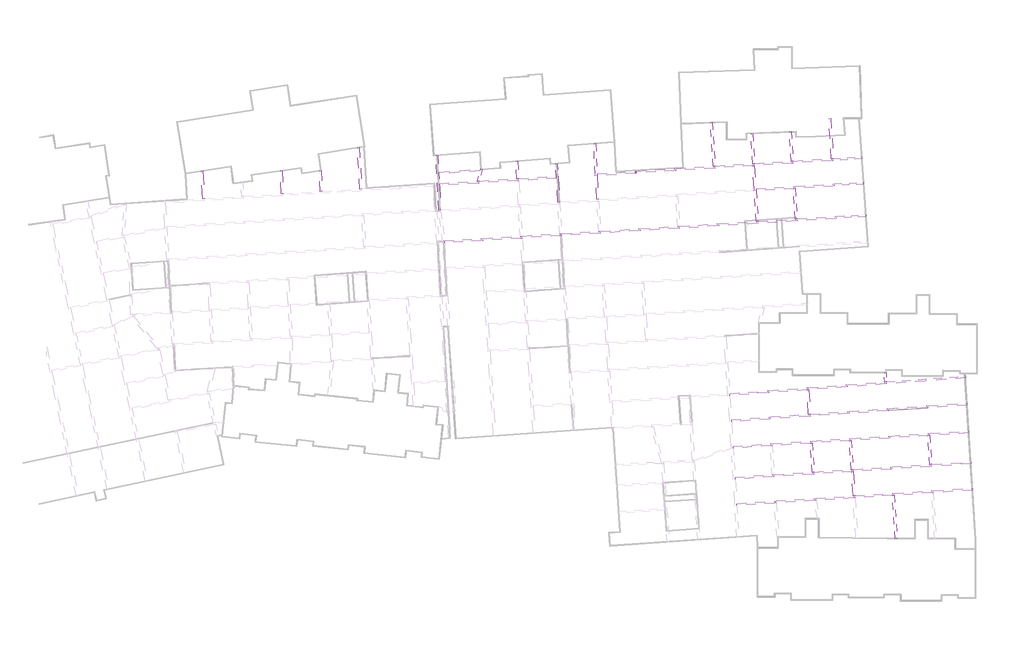
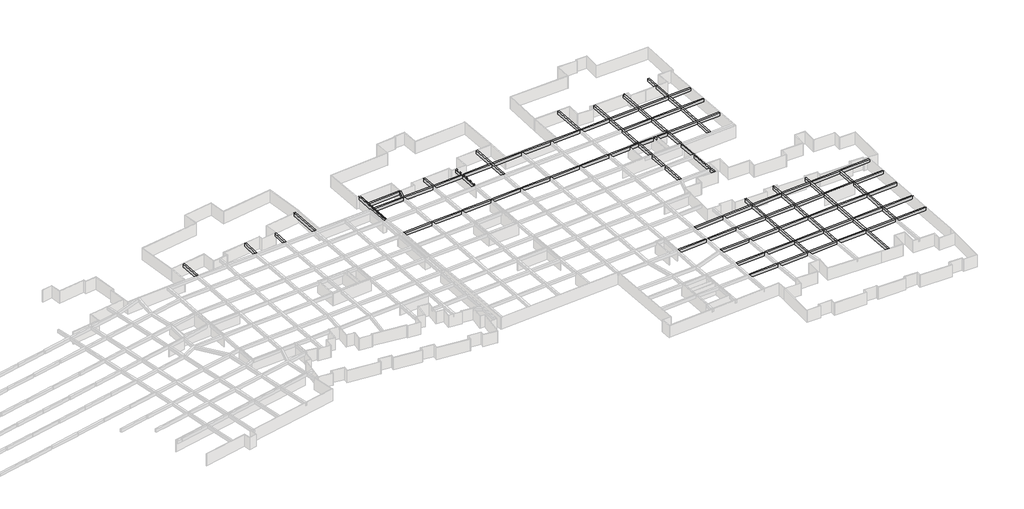
# One storey, part 14 of 14: 33 beams.
"""IFC4 building model written with IfcOpenShell, lengths in millimetres."""

from ifc_helpers import new_model, si_unit, frame, origin, place, context, project, spatial, polyline, outline, extrude, faceted_brep, element, save

model = new_model("IFC4")

# Units and contexts
model_context = context("Model", 3, world=origin())
ifc_project = project(units=[si_unit("LENGTHUNIT", "METRE", prefix="MILLI")], contexts=[model_context])

# Site, building, storey
site = spatial("IfcSite", under=ifc_project)
building = spatial("IfcBuilding", under=site)
storey = spatial("IfcBuildingStorey", under=building, Name="户型图", Elevation=0.0)

# Beams
placement = place(None, origin())
element("IfcBeam", 1, ObjectType="混凝土 - 矩形梁 : KL_beam", at=placement, inside=storey, context=model_context, shape_type="SweptSolid", body=[
    extrude(outline(polyline([(-187005.0921828, -124380.2167121), (-186605.8707912, -124355.2711605), (-186253.1826967, -129999.5894137), (-186652.4040882, -130024.5349652), (-187005.0921828, -124380.2167121)])), frame((0.0, 0.0, 2500.0), z_axis=(0.0, 0.0, 1.0), x_axis=(1.0, 0.0, 0.0)), (0.0, 0.0, 1.0), 800.0),
])
element("IfcBeam", 2, ObjectType="混凝土 - 矩形梁 : KL_beam", at=placement, inside=storey, context=model_context, shape_type="SweptSolid", body=[
    extrude(outline(polyline([(-170857.4371992, -124339.2940821), (-170457.6808684, -124325.3342834), (-170294.3543471, -129002.3939138), (-170693.7267176, -129027.3488993), (-170857.4371992, -124339.2940821)])), frame((0.0, 0.0, 2500.0), z_axis=(0.0, 0.0, 1.0), x_axis=(1.0, 0.0, 0.0)), (0.0, 0.0, 1.0), 800.0),
])
element("IfcBeam", 3, ObjectType="混凝土 - 矩形梁 : KL_beam", at=placement, inside=storey, context=model_context, shape_type="SweptSolid", body=[
    extrude(outline(polyline([(-162964.5535143, -124279.8902248), (-162565.3321228, -124254.9446733), (-162299.8992046, -128502.8563213), (-162699.1205962, -128527.8018729), (-162964.5535143, -124279.8902248)])), frame((0.0, 0.0, 2500.0), z_axis=(0.0, 0.0, 1.0), x_axis=(1.0, 0.0, 0.0)), (0.0, 0.0, 1.0), 800.0),
])
element("IfcBeam", 4, ObjectType="混凝土 - 矩形梁 : KL_beam", at=placement, inside=storey, context=model_context, shape_type="SweptSolid", body=[
    extrude(outline(polyline([(-155213.0308783, -119595.1268602), (-154813.8094867, -119570.1813086), (-154286.932885, -128002.1620485), (-154686.1542765, -128027.1076001), (-155213.0308783, -119595.1268602)])), frame((0.0, 0.0, 2500.0), z_axis=(0.0, 0.0, 1.0), x_axis=(1.0, 0.0, 0.0)), (0.0, 0.0, 1.0), 800.0),
])
element("IfcBeam", 5, ObjectType="混凝土 - 矩形梁 : KL_beam", at=placement, inside=storey, context=model_context, shape_type="Brep", body=[
    faceted_brep([(-52374.3043839, -126618.4184989, 3300.0), (-52349.2555626, -127017.6334242, 3300.0), (-52349.2555626, -127017.6334242, 2500.0), (-52374.3043839, -126618.4184989, 2500.0), (-58173.9130136, -126982.3161169, 3300.0), (-58573.1279522, -127007.3649391, 3300.0), (-66248.800325, -127488.9765565, 3300.0), (-66648.0254552, -127514.0260182, 3300.0), (-74177.9187714, -127986.4906992, 3300.0), (-74150.0154686, -128385.5265194, 3300.0), (-66620.1221525, -127913.0618384, 3300.0), (-66220.8970222, -127888.0123768, 3300.0), (-58548.1823998, -127406.586344, 3300.0), (-58148.9674612, -127381.5375218, 3300.0), (-74150.0154686, -128385.5265194, 2500.0), (-66620.1221525, -127913.0618384, 2500.0), (-66220.8970222, -127888.0123768, 2500.0), (-58548.1823998, -127406.586344, 2500.0), (-58148.9674612, -127381.5375218, 2500.0), (-74177.9187714, -127986.4906992, 2500.0), (-66648.0254552, -127514.0260182, 2500.0), (-66248.800325, -127488.9765565, 2500.0), (-58573.1279522, -127007.3649391, 2500.0), (-58173.9130136, -126982.3161169, 2500.0)], [[[0, 1, 2, 3]], [[1, 0, 4, 5, 6, 7, 8, 9, 10, 11, 12, 13]], [[2, 1, 13, 12, 11, 10, 9, 14, 15, 16, 17, 18]], [[3, 2, 18, 17, 16, 15, 14, 19, 20, 21, 22, 23]], [[0, 3, 23, 22, 21, 20, 19, 8, 7, 6, 5, 4]], [[8, 19, 14, 9]]]),
])
element("IfcBeam", 6, ObjectType="混凝土 - 矩形梁 : KL_beam", at=placement, inside=storey, context=model_context, shape_type="Brep", body=[
    faceted_brep([(-51938.8314526, -133222.3446571, 3300.0), (-51913.8859011, -133621.5660486, 3300.0), (-51913.8859011, -133621.5660486, 2500.0), (-51938.8314526, -133222.3446571, 2500.0), (-57761.268311, -133586.1625832, 3300.0), (-58160.4897025, -133611.1081347, 3300.0), (-65787.374178, -134087.6778873, 3300.0), (-66186.6065264, -134112.6241234, 3300.0), (-73716.6359875, -134583.1418412, 3300.0), (-74115.868336, -134608.0880774, 3300.0), (-81725.5469195, -135083.582711, 3300.0), (-82124.7687178, -135108.5282879, 3300.0), (-89692.9705485, -135581.4312256, 3300.0), (-90092.1926208, -135606.3768197, 3300.0), (-97677.4119955, -136080.3431072, 3300.0), (-98076.6340678, -136105.2887013, 3300.0), (-105753.707815, -136584.9945559, 3300.0), (-106152.9326387, -136609.9403219, 3300.0), (-113651.9046068, -137078.5173964, 3300.0), (-114051.1259984, -137103.462948, 3300.0), (-121674.9817155, -137579.843447, 3300.0), (-122074.2065392, -137604.789213, 3300.0), (-129690.7407312, -138080.7122228, 3300.0), (-130089.9623439, -138105.6577881, 3300.0), (-137513.7217746, -138569.535169, 3300.0), (-137466.852736, -138967.3866603, 3300.0), (-130064.5965359, -138504.8529197, 3300.0), (-129665.3749232, -138479.9073544, 3300.0), (-122048.4315655, -138003.9587776, 3300.0), (-121649.210174, -137979.0132261, 3300.0), (-114026.1804468, -137502.6843395, 3300.0), (-113626.9590553, -137477.738788, 3300.0), (-106126.3316752, -137009.0582742, 3300.0), (-105727.1068515, -136984.1125082, 3300.0), (-98050.9512296, -136504.4640231, 3300.0), (-97651.7291573, -136479.518429, 3300.0), (-90066.5097827, -136005.5521415, 3300.0), (-89667.2877103, -135980.6065474, 3300.0), (-82099.2532336, -135507.7140669, 3300.0), (-81700.0314352, -135482.76849, 3300.0), (-74087.9649807, -135007.124649, 3300.0), (-73688.7326322, -134982.1784128, 3300.0), (-66158.7031711, -134511.6606951, 3300.0), (-65759.4708227, -134486.7144589, 3300.0), (-58135.544151, -134010.3295263, 3300.0), (-57736.3227594, -133985.3839747, 3300.0), (-137466.852736, -138967.3866603, 2500.0), (-130064.5965359, -138504.8529197, 2500.0), (-129665.3749232, -138479.9073544, 2500.0), (-122048.4315655, -138003.9587776, 2500.0), (-121649.210174, -137979.0132261, 2500.0), (-114026.1804468, -137502.6843395, 2500.0), (-113626.9590553, -137477.738788, 2500.0), (-106126.3316752, -137009.0582742, 2500.0), (-105727.1068515, -136984.1125082, 2500.0), (-98050.9512296, -136504.4640231, 2500.0), (-97651.7291573, -136479.518429, 2500.0), (-90066.5097827, -136005.5521415, 2500.0), (-89667.2877103, -135980.6065474, 2500.0), (-82099.2532336, -135507.7140669, 2500.0), (-81700.0314352, -135482.76849, 2500.0), (-74087.9649807, -135007.124649, 2500.0), (-73688.7326322, -134982.1784128, 2500.0), (-66158.7031711, -134511.6606951, 2500.0), (-65759.4708227, -134486.7144589, 2500.0), (-58135.544151, -134010.3295263, 2500.0), (-57736.3227594, -133985.3839747, 2500.0), (-137513.7217746, -138569.535169, 2500.0), (-130089.9623439, -138105.6577881, 2500.0), (-129690.7407312, -138080.7122228, 2500.0), (-122074.2065392, -137604.789213, 2500.0), (-121674.9817155, -137579.843447, 2500.0), (-114051.1259984, -137103.462948, 2500.0), (-113651.9046068, -137078.5173964, 2500.0), (-106152.9326387, -136609.9403219, 2500.0), (-105753.707815, -136584.9945559, 2500.0), (-98076.6340678, -136105.2887013, 2500.0), (-97677.4119955, -136080.3431072, 2500.0), (-90092.1926208, -135606.3768197, 2500.0), (-89692.9705485, -135581.4312256, 2500.0), (-82124.7687178, -135108.5282879, 2500.0), (-81725.5469195, -135083.582711, 2500.0), (-74115.868336, -134608.0880774, 2500.0), (-73716.6359875, -134583.1418412, 2500.0), (-66186.6065264, -134112.6241234, 2500.0), (-65787.374178, -134087.6778873, 2500.0), (-58160.4897025, -133611.1081347, 2500.0), (-57761.268311, -133586.1625832, 2500.0)], [[[0, 1, 2, 3]], [[1, 0, 4, 5, 6, 7, 8, 9, 10, 11, 12, 13, 14, 15, 16, 17, 18, 19, 20, 21, 22, 23, 24, 25, 26, 27, 28, 29, 30, 31, 32, 33, 34, 35, 36, 37, 38, 39, 40, 41, 42, 43, 44, 45]], [[2, 1, 45, 44, 43, 42, 41, 40, 39, 38, 37, 36, 35, 34, 33, 32, 31, 30, 29, 28, 27, 26, 25, 46, 47, 48, 49, 50, 51, 52, 53, 54, 55, 56, 57, 58, 59, 60, 61, 62, 63, 64, 65, 66]], [[3, 2, 66, 65, 64, 63, 62, 61, 60, 59, 58, 57, 56, 55, 54, 53, 52, 51, 50, 49, 48, 47, 46, 67, 68, 69, 70, 71, 72, 73, 74, 75, 76, 77, 78, 79, 80, 81, 82, 83, 84, 85, 86, 87]], [[0, 3, 87, 86, 85, 84, 83, 82, 81, 80, 79, 78, 77, 76, 75, 74, 73, 72, 71, 70, 69, 68, 67, 24, 23, 22, 21, 20, 19, 18, 17, 16, 15, 14, 13, 12, 11, 10, 9, 8, 7, 6, 5, 4]], [[25, 24, 67, 46]]]),
])
element("IfcBeam", 7, ObjectType="混凝土 - 矩形梁 : KL_beam", at=placement, inside=storey, context=model_context, shape_type="Brep", body=[
    faceted_brep([(-129842.1738274, -124027.4632209, 3300.0), (-130231.923834, -123937.491379, 3300.0), (-130326.1623243, -124345.7241266, 3300.0), (-130806.4572254, -126426.3188663, 3300.0), (-130389.9881583, -126400.5461175, 3300.0), (-129842.1738274, -124027.4632209, 2500.0), (-130389.9881583, -126400.5461175, 2500.0), (-130231.923834, -123937.491379, 2500.0), (-130806.4572254, -126426.3188663, 2500.0), (-130326.1623243, -124345.7241266, 2500.0)], [[[0, 1, 2, 3, 4]], [[5, 0, 4, 6]], [[7, 5, 6, 8, 9]], [[1, 7, 9, 8, 3, 2]], [[4, 3, 8, 6]], [[1, 0, 5, 7]]]),
])
element("IfcBeam", 8, ObjectType="混凝土 - 矩形梁 : KL_beam", at=placement, inside=storey, context=model_context, shape_type="SweptSolid", body=[
    extrude(outline(polyline([(-123047.7665845, -122325.8850296), (-122648.896806, -122295.8367384), (-122377.03025, -125904.6726724), (-122776.3022919, -125929.3812014), (-123047.7665845, -122325.8850296)])), frame((0.0, 0.0, 2500.0), z_axis=(0.0, 0.0, 1.0), x_axis=(1.0, 0.0, 0.0)), (0.0, 0.0, 1.0), 800.0),
])
element("IfcBeam", 9, ObjectType="混凝土 - 矩形梁 : KL_beam", at=placement, inside=storey, context=model_context, shape_type="Brep", body=[
    faceted_brep([(-114574.1543033, -122851.64996, 3300.0), (-114574.1543033, -122851.64996, 2500.0), (-114973.2688243, -122878.2506949, 2500.0), (-114973.2688243, -122878.2506949, 3300.0), (-114802.7997937, -125435.9494127, 3300.0), (-114776.1987592, -125835.0684284, 3300.0), (-114453.9509255, -130670.0397306, 3300.0), (-114054.8364044, -130643.4389957, 3300.0), (-114376.9579948, -125810.3618349, 3300.0), (-114403.5590293, -125411.2428193, 3300.0), (-114802.7997937, -125435.9494127, 2500.0), (-114776.1987592, -125835.0684284, 2500.0), (-114453.9509255, -130670.0397306, 2500.0), (-114403.5590293, -125411.2428193, 2500.0), (-114376.9579948, -125810.3618349, 2500.0), (-114054.8364044, -130643.4389957, 2500.0)], [[[0, 1, 2, 3]], [[0, 3, 4, 5, 6, 7, 8, 9]], [[3, 2, 10, 11, 12, 6, 5, 4]], [[2, 1, 13, 14, 15, 12, 11, 10]], [[1, 0, 9, 8, 7, 15, 14, 13]], [[7, 6, 12, 15]]]),
])
element("IfcBeam", 10, ObjectType="混凝土 - 矩形梁 : KL_beam", at=placement, inside=storey, context=model_context, shape_type="Brep", body=[
    faceted_brep([(-107176.9227789, -118773.8861583, 3300.0), (-106777.470965, -118752.9517758, 3300.0), (-106777.470965, -118752.9517758, 2500.0), (-107176.9227789, -118773.8861583, 2500.0), (-106853.5598144, -124944.0190844, 3300.0), (-106832.624498, -125343.488717, 3300.0), (-106580.971679, -130145.3105546, 3300.0), (-106181.8169664, -130118.707141, 3300.0), (-106433.3957536, -125318.2979156, 3300.0), (-106454.3316163, -124918.8178582, 3300.0), (-106181.8169664, -130118.707141, 2500.0), (-106433.3957536, -125318.2979156, 2500.0), (-106454.3316163, -124918.8178582, 2500.0), (-106580.971679, -130145.3105546, 2500.0), (-106832.624498, -125343.488717, 2500.0), (-106853.5598144, -124944.0190844, 2500.0)], [[[0, 1, 2, 3]], [[1, 0, 4, 5, 6, 7, 8, 9]], [[2, 1, 9, 8, 7, 10, 11, 12]], [[3, 2, 12, 11, 10, 13, 14, 15]], [[0, 3, 15, 14, 13, 6, 5, 4]], [[7, 6, 13, 10]]]),
])
element("IfcBeam", 11, ObjectType="混凝土 - 矩形梁 : KL_beam", at=placement, inside=storey, context=model_context, shape_type="Brep", body=[
    faceted_brep([(-31634.7856178, -166005.21398, 3300.0), (-31604.8822978, -166404.0946532, 3300.0), (-31604.8822978, -166404.0946532, 2500.0), (-31634.7856178, -166005.21398, 2500.0), (-47623.313796, -167203.8433097, 3300.0), (-48022.1944692, -167233.7466297, 3300.0), (-55561.2153478, -167798.9325831, 3300.0), (-55960.1119301, -167828.8370958, 3300.0), (-63527.0942157, -168396.1192624, 3300.0), (-63925.978016, -168426.0228168, 3300.0), (-71553.260966, -168997.8256086, 3300.0), (-71952.1673161, -169027.7308535, 3300.0), (-79519.6147606, -169595.0478922, 3300.0), (-79494.0977596, -169994.2573993, 3300.0), (-71926.7900008, -169426.9508326, 3300.0), (-71527.8836507, -169397.0455877, 3300.0), (-63897.65415, -168825.0218986, 3300.0), (-63498.7703497, -168795.1183442, 3300.0), (-55933.7711758, -168227.9848477, 3300.0), (-55534.8745936, -168198.0803351, 3300.0), (-47994.1941782, -167632.7699693, 3300.0), (-47595.2955182, -167602.8653009, 3300.0), (-39950.5556653, -167029.7537985, 3300.0), (-39551.6447709, -166999.8482129, 3300.0), (-79494.0977596, -169994.2573993, 2500.0), (-71926.7900008, -169426.9508326, 2500.0), (-71527.8836507, -169397.0455877, 2500.0), (-63897.65415, -168825.0218986, 2500.0), (-63498.7703497, -168795.1183442, 2500.0), (-55933.7711758, -168227.9848477, 2500.0), (-55534.8745936, -168198.0803351, 2500.0), (-47994.1941782, -167632.7699693, 2500.0), (-47595.2955182, -167602.8653009, 2500.0), (-39950.5556653, -167029.7537985, 2500.0), (-39551.6447709, -166999.8482129, 2500.0), (-79519.6147606, -169595.0478922, 2500.0), (-71952.1673161, -169027.7308535, 2500.0), (-71553.260966, -168997.8256086, 2500.0), (-63925.978016, -168426.0228168, 2500.0), (-63527.0942157, -168396.1192624, 2500.0), (-55960.1119301, -167828.8370958, 2500.0), (-55561.2153478, -167798.9325831, 2500.0), (-48022.1944692, -167233.7466297, 2500.0), (-47623.313796, -167203.8433097, 2500.0)], [[[0, 1, 2, 3]], [[1, 0, 4, 5, 6, 7, 8, 9, 10, 11, 12, 13, 14, 15, 16, 17, 18, 19, 20, 21, 22, 23]], [[2, 1, 23, 22, 21, 20, 19, 18, 17, 16, 15, 14, 13, 24, 25, 26, 27, 28, 29, 30, 31, 32, 33, 34]], [[3, 2, 34, 33, 32, 31, 30, 29, 28, 27, 26, 25, 24, 35, 36, 37, 38, 39, 40, 41, 42, 43]], [[0, 3, 43, 42, 41, 40, 39, 38, 37, 36, 35, 12, 11, 10, 9, 8, 7, 6, 5, 4]], [[12, 35, 24, 13]]]),
])
element("IfcBeam", 12, ObjectType="混凝土 - 矩形梁 : KL_beam", at=placement, inside=storey, context=model_context, shape_type="Brep", body=[
    faceted_brep([(-106832.624498, -125343.488717, 3300.0), (-106853.5598144, -124944.0190844, 3300.0), (-114403.5590293, -125411.2428193, 3300.0), (-114376.9579948, -125810.3618349, 3300.0), (-106832.624498, -125343.488717, 2500.0), (-114376.9579948, -125810.3618349, 2500.0), (-106853.5598144, -124944.0190844, 2500.0), (-114403.5590293, -125411.2428193, 2500.0)], [[[0, 1, 2, 3]], [[4, 0, 3, 5]], [[6, 4, 5, 7]], [[1, 6, 7, 2]], [[1, 0, 4, 6]], [[3, 2, 7, 5]]]),
    faceted_brep([(-114802.7997937, -125435.9494127, 3300.0), (-114776.1987592, -125835.0684284, 3300.0), (-114776.1987592, -125835.0684284, 2500.0), (-114802.7997937, -125435.9494127, 2500.0), (-122377.03025, -125904.6726724, 3300.0), (-122776.3022919, -125929.3812014, 3300.0), (-130389.9881583, -126400.5461175, 3300.0), (-130806.4572254, -126426.3188663, 3300.0), (-138525.1741329, -126903.9835175, 3300.0), (-138504.2388166, -127303.4531502, 3300.0), (-130806.6290639, -126827.0946929, 3300.0), (-130407.3922508, -126802.388344, 3300.0), (-122753.4617992, -126328.7329342, 3300.0), (-122354.2077216, -126304.0255169, 3300.0), (-138504.2388166, -127303.4531502, 2500.0), (-130806.6290639, -126827.0946929, 2500.0), (-130407.3922508, -126802.388344, 2500.0), (-122753.4617992, -126328.7329342, 2500.0), (-122354.2077216, -126304.0255169, 2500.0), (-138525.1741329, -126903.9835175, 2500.0), (-130806.4572254, -126426.3188663, 2500.0), (-130389.9881583, -126400.5461175, 2500.0), (-122776.3022919, -125929.3812014, 2500.0), (-122377.03025, -125904.6726724, 2500.0)], [[[0, 1, 2, 3]], [[1, 0, 4, 5, 6, 7, 8, 9, 10, 11, 12, 13]], [[2, 1, 13, 12, 11, 10, 9, 14, 15, 16, 17, 18]], [[3, 2, 18, 17, 16, 15, 14, 19, 20, 21, 22, 23]], [[0, 3, 23, 22, 21, 20, 19, 8, 7, 6, 5, 4]], [[9, 8, 19, 14]]]),
])
element("IfcBeam", 13, ObjectType="混凝土 - 矩形梁 : KL_beam", at=placement, inside=storey, context=model_context, shape_type="Brep", body=[
    faceted_brep([(-98647.1108371, -124817.3303339, 3300.0), (-98649.2821204, -124783.5831797, 3300.0), (-98672.7936315, -124418.1556929, 3300.0), (-98827.9389787, -124428.1377049, 3300.0), (-106454.3316163, -124918.8178582, 3300.0), (-106433.3957536, -125318.2979156, 3300.0), (-98802.2561843, -124827.3123459, 3300.0), (-98647.1108371, -124817.3303339, 2500.0), (-106433.3957536, -125318.2979156, 2500.0), (-98802.2561843, -124827.3123459, 2500.0), (-98672.7936315, -124418.1556929, 2500.0), (-98649.2821204, -124783.5831797, 2500.0), (-106454.3316163, -124918.8178582, 2500.0), (-98827.9389787, -124428.1377049, 2500.0)], [[[0, 1, 2, 3, 4, 5, 6]], [[7, 0, 6, 5, 8, 9]], [[10, 11, 7, 9, 8, 12, 13]], [[2, 10, 13, 12, 4, 3]], [[5, 4, 12, 8]], [[2, 1, 0, 7, 11, 10]]]),
])
element("IfcBeam", 14, ObjectType="混凝土 - 矩形梁 : KL_beam", at=placement, inside=storey, context=model_context, shape_type="SweptSolid", body=[
    extrude(outline(polyline([(-130231.923834, -123937.491379), (-130326.1623243, -124345.7241266), (-138626.4766377, -124971.0165776), (-138647.4164777, -124571.4606268), (-130231.923834, -123937.491379)])), frame((0.0, 0.0, 2500.0), z_axis=(0.0, 0.0, 1.0), x_axis=(1.0, 0.0, 0.0)), (0.0, 0.0, 1.0), 800.0),
])
element("IfcBeam", 15, ObjectType="混凝土 - 矩形梁 : KL_beam", at=placement, inside=storey, context=model_context, shape_type="Brep", body=[
    faceted_brep([(-52735.750442, -121456.1127854, 3300.0), (-52710.3049507, -121855.3026237, 3300.0), (-52710.3049507, -121855.3026237, 2500.0), (-52735.750442, -121456.1127854, 2500.0), (-58496.276443, -121823.3050331, 3300.0), (-58895.4665943, -121848.7505443, 3300.0), (-66607.5973218, -122340.3436063, 3300.0), (-67006.78716, -122365.7890976, 3300.0), (-74491.5966275, -122842.8920585, 3300.0), (-74890.7864658, -122868.3375498, 3300.0), (-82475.3933928, -123351.8018835, 3300.0), (-82874.5832311, -123377.2473747, 3300.0), (-90447.1281157, -123859.9428397, 3300.0), (-90846.3180245, -123885.3883354, 3300.0), (-98430.9262918, -124368.8527546, 3300.0), (-98674.8462654, -124384.4009048, 3300.0), (-98672.6950439, -124418.1493498, 3300.0), (-98649.4007742, -124783.590743, 3300.0), (-98405.2434928, -124768.0274662, 3300.0), (-90820.6352256, -124284.563047, 3300.0), (-90421.4453168, -124259.1175513, 3300.0), (-82849.1027592, -123776.4349832, 3300.0), (-82449.9129148, -123750.9894916, 3300.0), (-74908.6843946, -123270.2902204, 3300.0), (-74509.4869911, -123244.8442469, 3300.0), (-66980.1166378, -122764.9008489, 3300.0), (-66580.9192344, -122739.4548754, 3300.0), (-58870.5210232, -122247.9722489, 3300.0), (-58471.3308719, -122222.5267377, 3300.0), (-98649.4007742, -124783.590743, 2500.0), (-98405.2434928, -124768.0274662, 2500.0), (-90820.6352256, -124284.563047, 2500.0), (-90421.4453168, -124259.1175513, 2500.0), (-82849.1027592, -123776.4349832, 2500.0), (-82449.9129148, -123750.9894916, 2500.0), (-74908.6843946, -123270.2902204, 2500.0), (-74509.4869911, -123244.8442469, 2500.0), (-66980.1166378, -122764.9008489, 2500.0), (-66580.9192344, -122739.4548754, 2500.0), (-58870.5210232, -122247.9722489, 2500.0), (-58471.3308719, -122222.5267377, 2500.0), (-98672.6950439, -124418.1493498, 2500.0), (-98674.8462654, -124384.4009048, 2500.0), (-98430.9262918, -124368.8527546, 2500.0), (-90846.3180245, -123885.3883354, 2500.0), (-90447.1281157, -123859.9428397, 2500.0), (-82874.5832311, -123377.2473747, 2500.0), (-82475.3933928, -123351.8018835, 2500.0), (-74890.7864658, -122868.3375498, 2500.0), (-74491.5966275, -122842.8920585, 2500.0), (-67006.78716, -122365.7890976, 2500.0), (-66607.5973218, -122340.3436063, 2500.0), (-58895.4665943, -121848.7505443, 2500.0), (-58496.276443, -121823.3050331, 2500.0)], [[[0, 1, 2, 3]], [[1, 0, 4, 5, 6, 7, 8, 9, 10, 11, 12, 13, 14, 15, 16, 17, 18, 19, 20, 21, 22, 23, 24, 25, 26, 27, 28]], [[2, 1, 28, 27, 26, 25, 24, 23, 22, 21, 20, 19, 18, 17, 29, 30, 31, 32, 33, 34, 35, 36, 37, 38, 39, 40]], [[3, 2, 40, 39, 38, 37, 36, 35, 34, 33, 32, 31, 30, 29, 41, 42, 43, 44, 45, 46, 47, 48, 49, 50, 51, 52, 53]], [[0, 3, 53, 52, 51, 50, 49, 48, 47, 46, 45, 44, 43, 42, 15, 14, 13, 12, 11, 10, 9, 8, 7, 6, 5, 4]], [[15, 42, 41, 29, 17, 16]]]),
])
element("IfcBeam", 16, ObjectType="混凝土 - 矩形梁 : KL_beam", at=placement, inside=storey, context=model_context, shape_type="SweptSolid", body=[
    extrude(outline(polyline([(-83442.4636616, -114468.3174988), (-83043.2738233, -114442.8720075), (-82475.3933928, -123351.8018835), (-82874.5832311, -123377.2473747), (-83442.4636616, -114468.3174988)])), frame((0.0, 0.0, 2500.0), z_axis=(0.0, 0.0, 1.0), x_axis=(1.0, 0.0, 0.0)), (0.0, 0.0, 1.0), 800.0),
])
element("IfcBeam", 17, ObjectType="混凝土 - 矩形梁 : KL_beam", at=placement, inside=storey, context=model_context, shape_type="SweptSolid", body=[
    extrude(outline(polyline([(-75277.2537161, -116805.42457), (-74878.0638779, -116779.9790787), (-74491.5966275, -122842.8920585), (-74890.7864658, -122868.3375498), (-75277.2537161, -116805.42457)])), frame((0.0, 0.0, 2500.0), z_axis=(0.0, 0.0, 1.0), x_axis=(1.0, 0.0, 0.0)), (0.0, 0.0, 1.0), 800.0),
])
element("IfcBeam", 18, ObjectType="混凝土 - 矩形梁 : KL_beam", at=placement, inside=storey, context=model_context, shape_type="SweptSolid", body=[
    extrude(outline(polyline([(-67390.2618088, -116349.8241659), (-66991.0719705, -116324.3786746), (-66607.5973218, -122340.3436063), (-67006.78716, -122365.7890976), (-67390.2618088, -116349.8241659)])), frame((0.0, 0.0, 2500.0), z_axis=(0.0, 0.0, 1.0), x_axis=(1.0, 0.0, 0.0)), (0.0, 0.0, 1.0), 800.0),
])
element("IfcBeam", 19, ObjectType="混凝土 - 矩形梁 : KL_beam", at=placement, inside=storey, context=model_context, shape_type="SweptSolid", body=[
    extrude(outline(polyline([(-59405.2866368, -113689.7380459), (-59006.0652453, -113664.7924943), (-58496.276443, -121823.3050331), (-58895.4665943, -121848.7505443), (-59405.2866368, -113689.7380459)])), frame((0.0, 0.0, 2500.0), z_axis=(0.0, 0.0, 1.0), x_axis=(1.0, 0.0, 0.0)), (0.0, 0.0, 1.0), 800.0),
    extrude(outline(polyline([(-57425.127004, -138965.6708341), (-57824.3483955, -138990.6163857), (-58135.544151, -134010.3295263), (-57736.3227594, -133985.3839747), (-57425.127004, -138965.6708341)])), frame((0.0, 0.0, 2500.0), z_axis=(0.0, 0.0, 1.0), x_axis=(1.0, 0.0, 0.0)), (0.0, 0.0, 1.0), 800.0),
    extrude(outline(polyline([(-58548.1823998, -127406.586344), (-58148.9674612, -127381.5375218), (-57761.268311, -133586.1625832), (-58160.4897025, -133611.1081347), (-58548.1823998, -127406.586344)])), frame((0.0, 0.0, 2500.0), z_axis=(0.0, 0.0, 1.0), x_axis=(1.0, 0.0, 0.0)), (0.0, 0.0, 1.0), 800.0),
    extrude(outline(polyline([(-58173.9130136, -126982.3161169), (-58573.1279522, -127007.3649391), (-58870.5210232, -122247.9722489), (-58471.3308719, -122222.5267377), (-58173.9130136, -126982.3161169)])), frame((0.0, 0.0, 2500.0), z_axis=(0.0, 0.0, 1.0), x_axis=(1.0, 0.0, 0.0)), (0.0, 0.0, 1.0), 800.0),
])
element("IfcBeam", 20, ObjectType="混凝土 - 矩形梁 : KL_beam", at=placement, inside=storey, context=model_context, shape_type="SweptSolid", body=[
    extrude(outline(polyline([(-64460.4085886, -153064.1699143), (-64859.4342087, -153092.0725038), (-64959.6104423, -151659.4856204), (-64560.4102838, -151634.0790467), (-64460.4085886, -153064.1699143)])), frame((0.0, 0.0, 2500.0), z_axis=(0.0, 0.0, 1.0), x_axis=(1.0, 0.0, 0.0)), (0.0, 0.0, 1.0), 800.0),
    extrude(outline(polyline([(-66980.1166378, -122764.9008489), (-66580.9192344, -122739.4548754), (-66248.800325, -127488.9765565), (-66648.0254552, -127514.0260182), (-66980.1166378, -122764.9008489)])), frame((0.0, 0.0, 2500.0), z_axis=(0.0, 0.0, 1.0), x_axis=(1.0, 0.0, 0.0)), (0.0, 0.0, 1.0), 800.0),
    extrude(outline(polyline([(-66620.1221525, -127913.0618384), (-66220.8970222, -127888.0123768), (-65787.374178, -134087.6778873), (-66186.6065264, -134112.6241234), (-66620.1221525, -127913.0618384)])), frame((0.0, 0.0, 2500.0), z_axis=(0.0, 0.0, 1.0), x_axis=(1.0, 0.0, 0.0)), (0.0, 0.0, 1.0), 800.0),
    extrude(outline(polyline([(-66158.7031711, -134511.6606951), (-65759.4708227, -134486.7144589), (-65411.3764652, -139464.6956904), (-65810.6088137, -139489.6419266), (-66158.7031711, -134511.6606951)])), frame((0.0, 0.0, 2500.0), z_axis=(0.0, 0.0, 1.0), x_axis=(1.0, 0.0, 0.0)), (0.0, 0.0, 1.0), 800.0),
    extrude(outline(polyline([(-65782.7054584, -139888.6784983), (-65383.4731099, -139863.7322621), (-65042.807434, -144735.4783979), (-65442.0397825, -144760.4246341), (-65782.7054584, -139888.6784983)])), frame((0.0, 0.0, 2500.0), z_axis=(0.0, 0.0, 1.0), x_axis=(1.0, 0.0, 0.0)), (0.0, 0.0, 1.0), 800.0),
    extrude(outline(polyline([(-65414.1364272, -145159.4612058), (-65014.9040787, -145134.5149696), (-64588.3134192, -151235.04562), (-64987.5135777, -151260.4521937), (-65414.1364272, -145159.4612058)])), frame((0.0, 0.0, 2500.0), z_axis=(0.0, 0.0, 1.0), x_axis=(1.0, 0.0, 0.0)), (0.0, 0.0, 1.0), 800.0),
])
element("IfcBeam", 21, ObjectType="混凝土 - 矩形梁 : KL_beam", at=placement, inside=storey, context=model_context, shape_type="Brep", body=[
    faceted_brep([(-74509.4869911, -123244.8442469, 3300.0), (-74908.6843946, -123270.2902204, 3300.0), (-74577.0927331, -128012.2719042, 3300.0), (-74549.1899952, -128411.2996475, 3300.0), (-74115.868336, -134608.0880774, 3300.0), (-73716.6359875, -134583.1418412, 3300.0), (-74150.0154686, -128385.5265194, 3300.0), (-74177.9187714, -127986.4906992, 3300.0), (-74509.4869911, -123244.8442469, 2500.0), (-73716.6359875, -134583.1418412, 2500.0), (-74150.0154686, -128385.5265194, 2500.0), (-74177.9187714, -127986.4906992, 2500.0), (-74908.6843946, -123270.2902204, 2500.0), (-74115.868336, -134608.0880774, 2500.0), (-74549.1899952, -128411.2996475, 2500.0), (-74577.0927331, -128012.2719042, 2500.0)], [[[0, 1, 2, 3, 4, 5, 6, 7]], [[8, 0, 7, 6, 5, 9, 10, 11]], [[12, 8, 11, 10, 9, 13, 14, 15]], [[1, 12, 15, 14, 13, 4, 3, 2]], [[1, 0, 8, 12]], [[5, 4, 13, 9]]]),
    faceted_brep([(-72516.9358957, -151739.652462, 3300.0), (-72916.1360542, -151765.0590358, 3300.0), (-72916.1360542, -151765.0590358, 2500.0), (-72516.9358957, -151739.652462, 2500.0), (-73343.3982367, -145654.9251597, 3300.0), (-72944.1658883, -145629.9789235, 3300.0), (-72944.1658883, -145629.9789235, 2500.0), (-73343.3982367, -145654.9251597, 2500.0)], [[[0, 1, 2, 3]], [[4, 5, 6, 7]], [[1, 0, 5, 4]], [[0, 3, 6, 5]], [[3, 2, 7, 6]], [[2, 1, 4, 7]]]),
    faceted_brep([(-74087.9649807, -135007.124649, 3300.0), (-73688.7326322, -134982.1784128, 3300.0), (-73688.7326322, -134982.1784128, 2500.0), (-74087.9649807, -135007.124649, 2500.0), (-73739.8706232, -139985.1058805, 3300.0), (-73340.6382748, -139960.1596443, 3300.0), (-73340.6382748, -139960.1596443, 2500.0), (-73739.8706232, -139985.1058805, 2500.0)], [[[0, 1, 2, 3]], [[1, 0, 4, 5]], [[2, 1, 5, 6]], [[3, 2, 6, 7]], [[0, 3, 7, 4]], [[5, 4, 7, 6]]]),
    faceted_brep([(-73711.9672679, -140384.1424522, 3300.0), (-73312.7349195, -140359.196216, 3300.0), (-73312.7349195, -140359.196216, 2500.0), (-73711.9672679, -140384.1424522, 2500.0), (-73371.301592, -145255.888588, 3300.0), (-72972.0692436, -145230.9423519, 3300.0), (-72972.0692436, -145230.9423519, 2500.0), (-73371.301592, -145255.888588, 2500.0)], [[[0, 1, 2, 3]], [[1, 0, 4, 5]], [[2, 1, 5, 6]], [[3, 2, 6, 7]], [[0, 3, 7, 4]], [[5, 4, 7, 6]]]),
])
element("IfcBeam", 22, ObjectType="混凝土 - 矩形梁 : KL_beam", at=placement, inside=storey, context=model_context, shape_type="Brep", body=[
    faceted_brep([(-31387.4075933, -171514.3760389, 3300.0), (-31359.0839494, -171913.3719928, 3300.0), (-31359.0839494, -171913.3719928, 2500.0), (-31387.4075933, -171514.3760389, 2500.0), (-39234.1642284, -172071.3960757, 3300.0), (-39633.1740911, -172099.720707, 3300.0), (-47265.6421941, -172641.5289803, 3300.0), (-47664.6442638, -172669.8530584, 3300.0), (-55204.4499854, -173205.0834798, 3300.0), (-55603.45087, -173233.4074737, 3300.0), (-63145.7013251, -173768.8114402, 3300.0), (-63544.697279, -173797.1350841, 3300.0), (-71213.5765068, -174341.5280847, 3300.0), (-71612.5833458, -174369.8525013, 3300.0), (-79180.0779467, -174907.0484814, 3300.0), (-79154.5618568, -175306.243736, 3300.0), (-71587.2069717, -174769.0576739, 3300.0), (-71188.2001327, -174740.7332573, 3300.0), (-63517.5723178, -174196.2161292, 3300.0), (-63118.5692047, -174167.8919771, 3300.0), (-55577.1108407, -173632.544239, 3300.0), (-55178.1099561, -173604.2202451, 3300.0), (-47638.5297922, -173069.0058354, 3300.0), (-47239.5277224, -173040.6817573, 3300.0), (-39608.18201, -172498.9531595, 3300.0), (-39209.1721473, -172470.6285282, 3300.0), (-79154.5618568, -175306.243736, 2500.0), (-71587.2069717, -174769.0576739, 2500.0), (-71188.2001327, -174740.7332573, 2500.0), (-63517.5723178, -174196.2161292, 2500.0), (-63118.5692047, -174167.8919771, 2500.0), (-55577.1108407, -173632.544239, 2500.0), (-55178.1099561, -173604.2202451, 2500.0), (-47638.5297922, -173069.0058354, 2500.0), (-47239.5277224, -173040.6817573, 2500.0), (-39608.18201, -172498.9531595, 2500.0), (-39209.1721473, -172470.6285282, 2500.0), (-79180.0779467, -174907.0484814, 2500.0), (-71612.5833458, -174369.8525013, 2500.0), (-71213.5765068, -174341.5280847, 2500.0), (-63544.697279, -173797.1350841, 2500.0), (-63145.7013251, -173768.8114402, 2500.0), (-55603.45087, -173233.4074737, 2500.0), (-55204.4499854, -173205.0834798, 2500.0), (-47664.6442638, -172669.8530584, 2500.0), (-47265.6421941, -172641.5289803, 2500.0), (-39633.1740911, -172099.720707, 2500.0), (-39234.1642284, -172071.3960757, 2500.0)], [[[0, 1, 2, 3]], [[1, 0, 4, 5, 6, 7, 8, 9, 10, 11, 12, 13, 14, 15, 16, 17, 18, 19, 20, 21, 22, 23, 24, 25]], [[2, 1, 25, 24, 23, 22, 21, 20, 19, 18, 17, 16, 15, 26, 27, 28, 29, 30, 31, 32, 33, 34, 35, 36]], [[3, 2, 36, 35, 34, 33, 32, 31, 30, 29, 28, 27, 26, 37, 38, 39, 40, 41, 42, 43, 44, 45, 46, 47]], [[0, 3, 47, 46, 45, 44, 43, 42, 41, 40, 39, 38, 37, 14, 13, 12, 11, 10, 9, 8, 7, 6, 5, 4]], [[15, 14, 37, 26]]]),
    faceted_brep([(-87136.6712903, -175872.8721019, 2500.0), (-87136.6712903, -175872.8721019, 3300.0), (-87159.6399867, -175476.127561, 3300.0), (-87159.7917111, -175473.5067853, 3300.0), (-87159.7917111, -175473.5067853, 2500.0), (-87159.6399867, -175476.127561, 2500.0), (-79579.0837782, -174935.3728265, 3300.0), (-79553.5676883, -175334.5680811, 3300.0), (-79553.5676883, -175334.5680811, 2500.0), (-79579.0837782, -174935.3728265, 2500.0)], [[[0, 1, 2, 3, 4, 5]], [[6, 7, 8, 9]], [[3, 2, 1, 7, 6]], [[1, 0, 8, 7]], [[0, 5, 4, 9, 8]], [[4, 3, 6, 9]]]),
])
element("IfcBeam", 23, ObjectType="混凝土 - 矩形梁 : KL_beam", at=placement, inside=storey, context=model_context, shape_type="Brep", body=[
    faceted_brep([(-31018.2640275, -177175.8953577, 3300.0), (-30992.3310551, -177575.0538236, 3300.0), (-30992.3310551, -177575.0538236, 2500.0), (-31018.2640275, -177175.8953577, 2500.0), (-38882.6358266, -177686.8366351, 3300.0), (-39281.7954034, -177712.7696796, 3300.0), (-46901.4694294, -178207.8131591, 3300.0), (-47300.6279364, -178233.7461342, 3300.0), (-54840.269995, -178723.5900076, 3300.0), (-55239.4286682, -178749.5229935, 3300.0), (-62789.037897, -179240.0144251, 3300.0), (-63188.196363, -179265.9473975, 3300.0), (-70868.8244382, -179764.9510077, 3300.0), (-71267.9832931, -179790.8840053, 3300.0), (-78836.4788748, -180282.6024667, 3300.0), (-78810.9634026, -180681.7880572, 3300.0), (-71242.6075866, -180190.0786764, 3300.0), (-70843.4487316, -180164.1456787, 3300.0), (-63162.2633906, -179665.1058635, 3300.0), (-62763.1049247, -179639.1728911, 3300.0), (-55213.0889508, -179148.6550335, 3300.0), (-54813.9302776, -179122.7220477, 3300.0), (-47274.5138624, -178632.8928341, 3300.0), (-46875.3553554, -178606.9598591, 3300.0), (-39256.8041239, -178111.9893265, 3300.0), (-38857.6445471, -178086.056282, 3300.0), (-78810.9634026, -180681.7880572, 2500.0), (-71242.6075866, -180190.0786764, 2500.0), (-70843.4487316, -180164.1456787, 2500.0), (-63162.2633906, -179665.1058635, 2500.0), (-62763.1049247, -179639.1728911, 2500.0), (-55213.0889508, -179148.6550335, 2500.0), (-54813.9302776, -179122.7220477, 2500.0), (-47274.5138624, -178632.8928341, 2500.0), (-46875.3553554, -178606.9598591, 2500.0), (-39256.8041239, -178111.9893265, 2500.0), (-38857.6445471, -178086.056282, 2500.0), (-78836.4788748, -180282.6024667, 2500.0), (-71267.9832931, -179790.8840053, 2500.0), (-70868.8244382, -179764.9510077, 2500.0), (-63188.196363, -179265.9473975, 2500.0), (-62789.037897, -179240.0144251, 2500.0), (-55239.4286682, -178749.5229935, 2500.0), (-54840.269995, -178723.5900076, 2500.0), (-47300.6279364, -178233.7461342, 2500.0), (-46901.4694294, -178207.8131591, 2500.0), (-39281.7954034, -177712.7696796, 2500.0), (-38882.6358266, -177686.8366351, 2500.0)], [[[0, 1, 2, 3]], [[1, 0, 4, 5, 6, 7, 8, 9, 10, 11, 12, 13, 14, 15, 16, 17, 18, 19, 20, 21, 22, 23, 24, 25]], [[2, 1, 25, 24, 23, 22, 21, 20, 19, 18, 17, 16, 15, 26, 27, 28, 29, 30, 31, 32, 33, 34, 35, 36]], [[3, 2, 36, 35, 34, 33, 32, 31, 30, 29, 28, 27, 26, 37, 38, 39, 40, 41, 42, 43, 44, 45, 46, 47]], [[0, 3, 47, 46, 45, 44, 43, 42, 41, 40, 39, 38, 37, 14, 13, 12, 11, 10, 9, 8, 7, 6, 5, 4]], [[15, 14, 37, 26]]]),
])
element("IfcBeam", 24, ObjectType="混凝土 - 矩形梁 : KL_beam", at=placement, inside=storey, context=model_context, shape_type="Brep", body=[
    faceted_brep([(-30509.3950119, -183461.2648082, 3300.0), (-30483.4620396, -183860.4232742, 3300.0), (-30483.4620396, -183860.4232742, 2500.0), (-30509.3950119, -183461.2648082, 2500.0), (-38488.7022064, -183979.6733366, 3300.0), (-38887.8617832, -184005.6063811, 3300.0), (-46489.8373745, -184499.500009, 3300.0), (-46888.9958815, -184525.4329841, 3300.0), (-54425.081159, -185015.0457766, 3300.0), (-54824.2398322, -185040.9787624, 3300.0), (-62380.2605197, -185531.8867409, 3300.0), (-62779.4189857, -185557.8197133, 3300.0), (-70468.8311543, -186057.3940182, 3300.0), (-70867.9900093, -186083.3270159, 3300.0), (-78434.2824865, -186574.9023435, 3300.0), (-78408.7670142, -186974.087934, 3300.0), (-70842.6143027, -186482.5216869, 3300.0), (-70443.4554478, -186456.5886893, 3300.0), (-62753.4860133, -185956.9781792, 3300.0), (-62354.3275474, -185931.0452069, 3300.0), (-54798.1033837, -185440.1240087, 3300.0), (-54398.9449178, -185414.1910363, 3300.0), (-46862.8818075, -184924.579684, 3300.0), (-46463.7233005, -184898.646709, 3300.0), (-38862.8705037, -184404.826028, 3300.0), (-38463.710927, -184378.8929835, 3300.0), (-78408.7670142, -186974.087934, 2500.0), (-70842.6143027, -186482.5216869, 2500.0), (-70443.4554478, -186456.5886893, 2500.0), (-62753.4860133, -185956.9781792, 2500.0), (-62354.3275474, -185931.0452069, 2500.0), (-54798.1033837, -185440.1240087, 2500.0), (-54398.9449178, -185414.1910363, 2500.0), (-46862.8818075, -184924.579684, 2500.0), (-46463.7233005, -184898.646709, 2500.0), (-38862.8705037, -184404.826028, 2500.0), (-38463.710927, -184378.8929835, 2500.0), (-78434.2824865, -186574.9023435, 2500.0), (-70867.9900093, -186083.3270159, 2500.0), (-70468.8311543, -186057.3940182, 2500.0), (-62779.4189857, -185557.8197133, 2500.0), (-62380.2605197, -185531.8867409, 2500.0), (-54824.2398322, -185040.9787624, 2500.0), (-54425.081159, -185015.0457766, 2500.0), (-46888.9958815, -184525.4329841, 2500.0), (-46489.8373745, -184499.500009, 2500.0), (-38887.8617832, -184005.6063811, 2500.0), (-38488.7022064, -183979.6733366, 2500.0)], [[[0, 1, 2, 3]], [[1, 0, 4, 5, 6, 7, 8, 9, 10, 11, 12, 13, 14, 15, 16, 17, 18, 19, 20, 21, 22, 23, 24, 25]], [[2, 1, 25, 24, 23, 22, 21, 20, 19, 18, 17, 16, 15, 26, 27, 28, 29, 30, 31, 32, 33, 34, 35, 36]], [[3, 2, 36, 35, 34, 33, 32, 31, 30, 29, 28, 27, 26, 37, 38, 39, 40, 41, 42, 43, 44, 45, 46, 47]], [[0, 3, 47, 46, 45, 44, 43, 42, 41, 40, 39, 38, 37, 14, 13, 12, 11, 10, 9, 8, 7, 6, 5, 4]], [[15, 14, 37, 26]]]),
])
element("IfcBeam", 25, ObjectType="混凝土 - 矩形梁 : KL_beam", at=placement, inside=storey, context=model_context, shape_type="Brep", body=[
    faceted_brep([(-30262.0915433, -188816.3990351, 3300.0), (-30236.1585709, -189215.5575011, 3300.0), (-30236.1585709, -189215.5575011, 2500.0), (-30262.0915433, -188816.3990351, 2500.0), (-38153.8252347, -189329.1179904, 3300.0), (-38552.9848114, -189355.0510349, 3300.0), (-46139.9152329, -189847.9671915, 3300.0), (-46539.0737399, -189873.9001665, 3300.0), (-54077.3824665, -190363.6574146, 3300.0), (-54476.5409324, -190389.5903869, 3300.0), (-62032.7650961, -190880.5115851, 3300.0), (-62431.923562, -190906.4445575, 3300.0), (-70128.8029548, -191406.5040014, 3300.0), (-70527.9618097, -191432.436999, 3300.0), (-78092.3814613, -191923.8906508, 3300.0), (-78066.8659891, -192323.0762413, 3300.0), (-70497.8882735, -191831.3264562, 3300.0), (-70098.6297483, -191805.3869831, 3300.0), (-62381.3788239, -191304.0040188, 3300.0), (-61978.7583486, -191277.8461227, 3300.0), (-54450.6079601, -190788.7488529, 3300.0), (-54051.4494941, -190762.8158805, 3300.0), (-46512.9596659, -190273.0468665, 3300.0), (-46113.8011588, -190247.1138914, 3300.0), (-38527.5221301, -189754.2400553, 3300.0), (-38128.3636641, -189728.3070829, 3300.0), (-78066.8659891, -192323.0762413, 2500.0), (-70497.8882735, -191831.3264562, 2500.0), (-70098.6297483, -191805.3869831, 2500.0), (-62381.3788239, -191304.0040188, 2500.0), (-61978.7583486, -191277.8461227, 2500.0), (-54450.6079601, -190788.7488529, 2500.0), (-54051.4494941, -190762.8158805, 2500.0), (-46512.9596659, -190273.0468665, 2500.0), (-46113.8011588, -190247.1138914, 2500.0), (-38527.5221301, -189754.2400553, 2500.0), (-38128.3636641, -189728.3070829, 2500.0), (-78092.3814613, -191923.8906508, 2500.0), (-70527.9618097, -191432.436999, 2500.0), (-70128.8029548, -191406.5040014, 2500.0), (-62431.923562, -190906.4445575, 2500.0), (-62032.7650961, -190880.5115851, 2500.0), (-54476.5409324, -190389.5903869, 2500.0), (-54077.3824665, -190363.6574146, 2500.0), (-46539.0737399, -189873.9001665, 2500.0), (-46139.9152329, -189847.9671915, 2500.0), (-38552.9848114, -189355.0510349, 2500.0), (-38153.8252347, -189329.1179904, 2500.0)], [[[0, 1, 2, 3]], [[1, 0, 4, 5, 6, 7, 8, 9, 10, 11, 12, 13, 14, 15, 16, 17, 18, 19, 20, 21, 22, 23, 24, 25]], [[2, 1, 25, 24, 23, 22, 21, 20, 19, 18, 17, 16, 15, 26, 27, 28, 29, 30, 31, 32, 33, 34, 35, 36]], [[3, 2, 36, 35, 34, 33, 32, 31, 30, 29, 28, 27, 26, 37, 38, 39, 40, 41, 42, 43, 44, 45, 46, 47]], [[0, 3, 47, 46, 45, 44, 43, 42, 41, 40, 39, 38, 37, 14, 13, 12, 11, 10, 9, 8, 7, 6, 5, 4]], [[15, 14, 37, 26]]]),
])
element("IfcBeam", 26, ObjectType="混凝土 - 矩形梁 : KL_beam", at=placement, inside=storey, context=model_context, shape_type="SweptSolid", body=[
    extrude(outline(polyline([(-64112.9012332, -165792.830295), (-63713.9052794, -165764.5066511), (-63527.0942157, -168396.1192624), (-63925.978016, -168426.0228168), (-64112.9012332, -165792.830295)])), frame((0.0, 0.0, 2500.0), z_axis=(0.0, 0.0, 1.0), x_axis=(1.0, 0.0, 0.0)), (0.0, 0.0, 1.0), 800.0),
    extrude(outline(polyline([(-63145.7013251, -173768.8114402), (-63544.697279, -173797.1350841), (-63897.65415, -168825.0218986), (-63498.7703497, -168795.1183442), (-63145.7013251, -173768.8114402)])), frame((0.0, 0.0, 2500.0), z_axis=(0.0, 0.0, 1.0), x_axis=(1.0, 0.0, 0.0)), (0.0, 0.0, 1.0), 800.0),
])
element("IfcBeam", 27, ObjectType="混凝土 - 矩形梁 : KL_beam", at=placement, inside=storey, context=model_context, shape_type="SweptSolid", body=[
    extrude(outline(polyline([(-62032.7650961, -190880.5115851), (-62431.923562, -190906.4445575), (-62753.4860133, -185956.9781792), (-62354.3275474, -185931.0452069), (-62032.7650961, -190880.5115851)])), frame((0.0, 0.0, 2500.0), z_axis=(0.0, 0.0, 1.0), x_axis=(1.0, 0.0, 0.0)), (0.0, 0.0, 1.0), 800.0),
    extrude(outline(polyline([(-63517.5723178, -174196.2161292), (-63118.5692047, -174167.8919771), (-62789.037897, -179240.0144251), (-63188.196363, -179265.9473975), (-63517.5723178, -174196.2161292)])), frame((0.0, 0.0, 2500.0), z_axis=(0.0, 0.0, 1.0), x_axis=(1.0, 0.0, 0.0)), (0.0, 0.0, 1.0), 800.0),
    extrude(outline(polyline([(-63162.2633906, -179665.1058635), (-62763.1049247, -179639.1728911), (-62380.2605197, -185531.8867409), (-62779.4189857, -185557.8197133), (-63162.2633906, -179665.1058635)])), frame((0.0, 0.0, 2500.0), z_axis=(0.0, 0.0, 1.0), x_axis=(1.0, 0.0, 0.0)), (0.0, 0.0, 1.0), 800.0),
])
element("IfcBeam", 28, ObjectType="混凝土 - 矩形梁 : KL_beam", at=placement, inside=storey, context=model_context, shape_type="SweptSolid", body=[
    extrude(outline(polyline([(-54798.1033837, -185440.1240087), (-54398.9449178, -185414.1910363), (-54077.3824665, -190363.6574146), (-54476.5409324, -190389.5903869), (-54798.1033837, -185440.1240087)])), frame((0.0, 0.0, 2500.0), z_axis=(0.0, 0.0, 1.0), x_axis=(1.0, 0.0, 0.0)), (0.0, 0.0, 1.0), 800.0),
])
element("IfcBeam", 29, ObjectType="混凝土 - 矩形梁 : KL_beam", at=placement, inside=storey, context=model_context, shape_type="SweptSolid", body=[
    extrude(outline(polyline([(-56170.0743754, -164647.2259261), (-55770.9425426, -164620.8862223), (-55561.2153478, -167798.9325831), (-55960.1119301, -167828.8370958), (-56170.0743754, -164647.2259261)])), frame((0.0, 0.0, 2500.0), z_axis=(0.0, 0.0, 1.0), x_axis=(1.0, 0.0, 0.0)), (0.0, 0.0, 1.0), 800.0),
    extrude(outline(polyline([(-54425.081159, -185015.0457766), (-54824.2398322, -185040.9787624), (-55213.0889508, -179148.6550335), (-54813.9302776, -179122.7220477), (-54425.081159, -185015.0457766)])), frame((0.0, 0.0, 2500.0), z_axis=(0.0, 0.0, 1.0), x_axis=(1.0, 0.0, 0.0)), (0.0, 0.0, 1.0), 800.0),
    extrude(outline(polyline([(-55933.7711758, -168227.9848477), (-55534.8745936, -168198.0803351), (-55204.4499854, -173205.0834798), (-55603.45087, -173233.4074737), (-55933.7711758, -168227.9848477)])), frame((0.0, 0.0, 2500.0), z_axis=(0.0, 0.0, 1.0), x_axis=(1.0, 0.0, 0.0)), (0.0, 0.0, 1.0), 800.0),
    extrude(outline(polyline([(-55577.1108407, -173632.544239), (-55178.1099561, -173604.2202451), (-54840.269995, -178723.5900076), (-55239.4286682, -178749.5229935), (-55577.1108407, -173632.544239)])), frame((0.0, 0.0, 2500.0), z_axis=(0.0, 0.0, 1.0), x_axis=(1.0, 0.0, 0.0)), (0.0, 0.0, 1.0), 800.0),
])
element("IfcBeam", 30, ObjectType="混凝土 - 矩形梁 : KL_beam", at=placement, inside=storey, context=model_context, shape_type="SweptSolid", body=[
    extrude(outline(polyline([(-48162.9967558, -165355.5835724), (-47764.1160826, -165325.6802524), (-47623.313796, -167203.8433097), (-48022.1944692, -167233.7466297), (-48162.9967558, -165355.5835724)])), frame((0.0, 0.0, 2500.0), z_axis=(0.0, 0.0, 1.0), x_axis=(1.0, 0.0, 0.0)), (0.0, 0.0, 1.0), 800.0),
])
element("IfcBeam", 31, ObjectType="混凝土 - 矩形梁 : KL_beam", at=placement, inside=storey, context=model_context, shape_type="SweptSolid", body=[
    extrude(outline(polyline([(-45538.2683299, -199043.9806285), (-45937.4149887, -199070.0946999), (-46512.9596659, -190273.0468665), (-46113.8011588, -190247.1138914), (-45538.2683299, -199043.9806285)])), frame((0.0, 0.0, 2500.0), z_axis=(0.0, 0.0, 1.0), x_axis=(1.0, 0.0, 0.0)), (0.0, 0.0, 1.0), 800.0),
    extrude(outline(polyline([(-47994.1941782, -167632.7699693), (-47595.2955182, -167602.8653009), (-47265.6421941, -172641.5289803), (-47664.6442638, -172669.8530584), (-47994.1941782, -167632.7699693)])), frame((0.0, 0.0, 2500.0), z_axis=(0.0, 0.0, 1.0), x_axis=(1.0, 0.0, 0.0)), (0.0, 0.0, 1.0), 800.0),
    extrude(outline(polyline([(-47638.5297922, -173069.0058354), (-47239.5277224, -173040.6817573), (-46901.4694294, -178207.8131591), (-47300.6279364, -178233.7461342), (-47638.5297922, -173069.0058354)])), frame((0.0, 0.0, 2500.0), z_axis=(0.0, 0.0, 1.0), x_axis=(1.0, 0.0, 0.0)), (0.0, 0.0, 1.0), 800.0),
    extrude(outline(polyline([(-47274.5138624, -178632.8928341), (-46875.3553554, -178606.9598591), (-46489.8373745, -184499.500009), (-46888.9958815, -184525.4329841), (-47274.5138624, -178632.8928341)])), frame((0.0, 0.0, 2500.0), z_axis=(0.0, 0.0, 1.0), x_axis=(1.0, 0.0, 0.0)), (0.0, 0.0, 1.0), 800.0),
    extrude(outline(polyline([(-46862.8818075, -184924.579684), (-46463.7233005, -184898.646709), (-46139.9152329, -189847.9671915), (-46539.0737399, -189873.9001665), (-46862.8818075, -184924.579684)])), frame((0.0, 0.0, 2500.0), z_axis=(0.0, 0.0, 1.0), x_axis=(1.0, 0.0, 0.0)), (0.0, 0.0, 1.0), 800.0),
])
element("IfcBeam", 32, ObjectType="混凝土 - 矩形梁 : KL_beam", at=placement, inside=storey, context=model_context, shape_type="SweptSolid", body=[
    extrude(outline(polyline([(-39950.5556653, -167029.7537985), (-39551.6447709, -166999.8482129), (-39234.1642284, -172071.3960757), (-39633.1740911, -172099.720707), (-39950.5556653, -167029.7537985)])), frame((0.0, 0.0, 2500.0), z_axis=(0.0, 0.0, 1.0), x_axis=(1.0, 0.0, 0.0)), (0.0, 0.0, 1.0), 800.0),
    extrude(outline(polyline([(-38153.8252347, -189329.1179904), (-38552.9848114, -189355.0510349), (-38862.8705037, -184404.826028), (-38463.710927, -184378.8929835), (-38153.8252347, -189329.1179904)])), frame((0.0, 0.0, 2500.0), z_axis=(0.0, 0.0, 1.0), x_axis=(1.0, 0.0, 0.0)), (0.0, 0.0, 1.0), 800.0),
    extrude(outline(polyline([(-39608.18201, -172498.9531595), (-39209.1721473, -172470.6285282), (-38882.6358266, -177686.8366351), (-39281.7954034, -177712.7696796), (-39608.18201, -172498.9531595)])), frame((0.0, 0.0, 2500.0), z_axis=(0.0, 0.0, 1.0), x_axis=(1.0, 0.0, 0.0)), (0.0, 0.0, 1.0), 800.0),
    extrude(outline(polyline([(-39256.8041239, -178111.9893265), (-38857.6445471, -178086.056282), (-38488.7022064, -183979.6733366), (-38887.8617832, -184005.6063811), (-39256.8041239, -178111.9893265)])), frame((0.0, 0.0, 2500.0), z_axis=(0.0, 0.0, 1.0), x_axis=(1.0, 0.0, 0.0)), (0.0, 0.0, 1.0), 800.0),
])
element("IfcBeam", 33, ObjectType="混凝土 - 矩形梁 : KL_beam", at=placement, inside=storey, context=model_context, shape_type="Brep", body=[
    faceted_brep([(-139224.9350005, -121194.6797973, 3300.0), (-138825.4831866, -121173.7454148, 3300.0), (-138825.4831866, -121173.7454148, 2500.0), (-139224.9350005, -121194.6797973, 2500.0), (-138643.8583896, -132282.2820359, 3300.0), (-138257.4280169, -132256.5266916, 3300.0), (-138244.7036771, -132255.6786223, 3300.0), (-138504.2388166, -127303.4531502, 3300.0), (-138525.1741329, -126903.9835175, 3300.0), (-138626.4766377, -124971.0165776, 3300.0), (-138647.4164777, -124571.4606268, 3300.0), (-138244.7036771, -132255.6786223, 2500.0), (-138504.2388166, -127303.4531502, 2500.0), (-138525.1741329, -126903.9835175, 2500.0), (-138626.4766377, -124971.0165776, 2500.0), (-138647.4164777, -124571.4606268, 2500.0), (-138257.4280169, -132256.5266916, 2500.0), (-138643.8583896, -132282.2820359, 2500.0)], [[[0, 1, 2, 3]], [[1, 0, 4, 5, 6, 7, 8, 9, 10]], [[2, 1, 10, 9, 8, 7, 6, 11, 12, 13, 14, 15]], [[3, 2, 15, 14, 13, 12, 11, 16, 17]], [[0, 3, 17, 4]], [[5, 4, 17, 16, 11, 6]]]),
])

save(model, "model.ifc")

# Revit data of these elements
# Type "混凝土 - 矩形梁 : KL_beam"
#   Length [instance default] = 1524 mm
#   b = 400 mm
#   h = 800 mm
#   Structural Material [instance default] = 混凝土 - 现场浇注混凝土
#   Assembly Code = ""
# Elements 1, 2, 3, 4, 5, 6, 7, 8, 9, 10, 11, 12, 13, 14, 15, 16, 17, 18, 19, 20, 21, 22, 23, 24, 25, 26, 27, 28, 29, 30, 31, 32, 33 (IfcBeam, "混凝土 - 矩形梁 : KL_beam")
#   Comments = ""
#   Structural Material = none
#   Phase Created = 新构造
# Materials
#   "混凝土 - 现场浇注混凝土": class "混凝土", colour RGB 192 192 192, transparency 0
